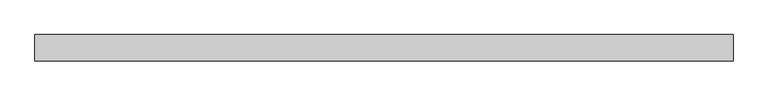
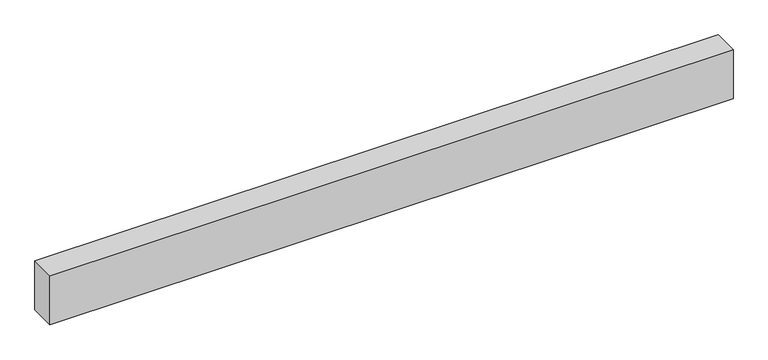
"""IFC4 building model written with IfcOpenShell, lengths in millimetres: beam geometry, Madeira de lei : Berço 6x12cm."""

from ifc_helpers import new_model, si_unit, frame, origin, place, context, project, spatial, polyline, outline, extrude, source, transform, mapped, element, save


def beam_c6e4bd39(model_context):
    return source(origin(), model_context, "Body", "SweptSolid", [
        extrude(outline(polyline([(789.5373463, 30.0), (789.5373463, -30.0), (-789.5373463, -30.0), (-789.5373463, 30.0), (789.5373463, 30.0)])), frame((0.0, 0.0, -60.0), z_axis=(0.0, 0.0, 1.0), x_axis=(1.0, 0.0, 0.0)), (0.0, 0.0, 1.0), 120.0),
    ])


if __name__ == "__main__":
    model = new_model("IFC4")
    model_context = context("Model", 3, world=origin())
    ifc_project = project(units=[si_unit("LENGTHUNIT", "METRE", prefix="MILLI")], contexts=[model_context])
    site = spatial("IfcSite", under=ifc_project)
    building = spatial("IfcBuilding", under=site)
    placement = place(None, origin())
    beam_shape = beam_c6e4bd39(model_context)
    element("IfcBeam", 1, ObjectType="Madeira de lei : Berço 6x12cm", at=placement, inside=building, context=model_context, shape_type="MappedRepresentation", body=[
        mapped(beam_shape, transform((0.0, 0.0, 0.0), x_axis=(1.0, 0.0, 0.0), y_axis=(0.0, 1.0, 0.0), z_axis=(0.0, 0.0, 1.0))),
    ])
    save(model, "model.ifc")

# Revit data of these elements
# Type "Madeira de lei : Berço 6x12cm"
#   A = 0.02 m²
#   Length [instance default] = 1.524 m
#   b = 0.06 m
#   d = 0.12 m
#   Structural Material [instance default] = none
#   Assembly Code = ""
# Element 1 (IfcBeam, "Madeira de lei : Berço 6x12cm")
#   Structural Material = .MADEIRAMENTO
#   Materials on its faces: ".MADEIRAMENTO"
# Materials
#   ".MADEIRAMENTO": class ".CC_MADEIRAS", colour RGB 212 179 113, transparency 0, Cost = 0
